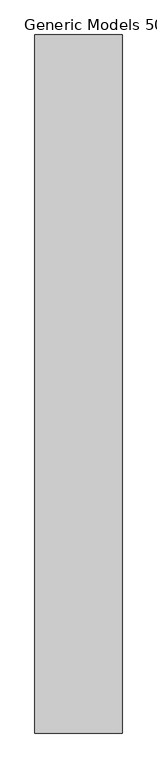
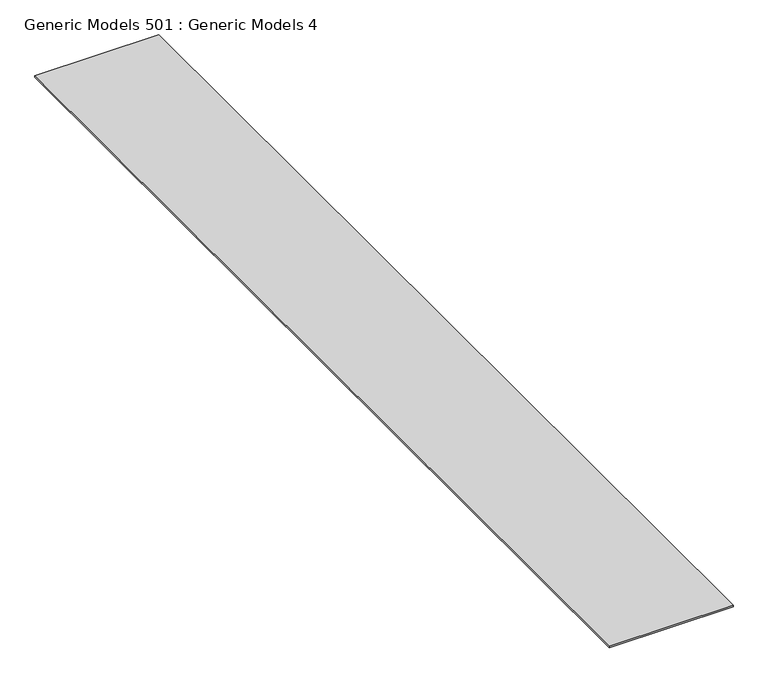
"""IFC4 building model written with IfcOpenShell, lengths in millimetres: proxy geometry, Generic Models 501 : Generic Models 4."""

import ifcopenshell
import ifcopenshell.guid

model = None  # the IFC model being written
_history = None  # IfcOwnerHistory: only IFC2X3 demands one
_inside = {}  # id of a spatial element -> (the spatial element, [elements in it])
_under = {}  # id of a project, library or spatial element -> (it, [spatial elements below it])
_declared = {}  # id of a project -> (the project, [libraries it declares])
_typed = {}  # id of a type object -> (the type object, [elements of that type])
_made_of = {}  # id of a material, layer set ... -> (it, [elements and type objects made of it])


def new_model(schema):
    """Start an empty IFC model of exactly this schema.

    Asked for "IFC4X3", IfcOpenShell would pick the latest addendum, in which some entities
    have other attributes; the version numbers below select the first issue.
    IFC2X3 requires an IfcOwnerHistory on every rooted entity: one is made here for all.
    """
    global model, _history
    if schema == "IFC4X3":
        model = ifcopenshell.file(schema_version=(4, 3, 0, 0))
    else:
        model = ifcopenshell.file(schema=schema)
    _inside.clear()
    _under.clear()
    _declared.clear()
    _typed.clear()
    _made_of.clear()
    _history = None
    if model.schema == "IFC2X3":
        org = make("IfcOrganization", Name="unknown")
        user = make(
            "IfcPersonAndOrganization",
            ThePerson=make("IfcPerson", FamilyName="unknown"),
            TheOrganization=org,
        )
        app = make(
            "IfcApplication",
            ApplicationDeveloper=org,
            Version="unknown",
            ApplicationFullName="unknown",
            ApplicationIdentifier="unknown",
        )
        _history = make(
            "IfcOwnerHistory",
            OwningUser=user,
            OwningApplication=app,
            ChangeAction="ADDED",
            CreationDate=0,
        )
    return model


def make(cls, **values):
    """One entity of the class cls with the attributes given. An attribute that is None is left unset."""
    return model.create_entity(
        cls, **{name: value for name, value in values.items() if value is not None}
    )


def rooted(cls, **values):
    """An entity with a GlobalId (a new one), such as an element, a storey or a relation."""
    return make(cls, GlobalId=ifcopenshell.guid.new(), OwnerHistory=_history, **values)


def si_unit(unit_type, name, prefix=None):
    """IfcSIUnit, for example si_unit("LENGTHUNIT", "METRE", prefix="MILLI")."""
    return make("IfcSIUnit", UnitType=unit_type, Prefix=prefix, Name=name)


def assignment(units):
    """IfcUnitAssignment: the units of a project."""
    return None if units is None else make("IfcUnitAssignment", Units=units)


def point(xyz):
    """IfcCartesianPoint."""
    return None if xyz is None else make("IfcCartesianPoint", Coordinates=xyz)


def direction(xyz):
    """IfcDirection."""
    return None if xyz is None else make("IfcDirection", DirectionRatios=xyz)


def frame(location, z_axis=None, x_axis=None):
    """IfcAxis2Placement3D, a coordinate frame: its origin and axes. An axis left out is left unset."""
    return make(
        "IfcAxis2Placement3D",
        Location=point(location),
        Axis=direction(z_axis),
        RefDirection=direction(x_axis),
    )


def origin():
    """The frame at (0, 0, 0) with its axes left unset."""
    return frame((0.0, 0.0, 0.0))


def place(relative_to, where):
    """IfcLocalPlacement: puts the frame where relative to a parent placement (None: the world)."""
    return make(
        "IfcLocalPlacement", PlacementRelTo=relative_to, RelativePlacement=where
    )


def context(
    kind, dimensions, precision=None, world=None, true_north=None, identifier=None
):
    """IfcGeometricRepresentationContext, for example the 3D "Model" context."""
    return make(
        "IfcGeometricRepresentationContext",
        ContextIdentifier=identifier,
        ContextType=kind,
        CoordinateSpaceDimension=dimensions,
        Precision=precision,
        WorldCoordinateSystem=world,
        TrueNorth=true_north,
    )


def project(units=None, contexts=None):
    """IfcProject with its units and contexts."""
    return rooted(
        "IfcProject",
        Name="project",
        RepresentationContexts=contexts,
        UnitsInContext=assignment(units),
    )


def spatial(cls, under=None, at=None, **own):
    """A site, building, storey or space (cls), placed at a placement, below another one or the project."""
    s = rooted(cls, ObjectPlacement=at, **own)
    if under is not None:
        _under.setdefault(under.id(), (under, []))[1].append(s)
    return s


def polyline(points):
    """IfcPolyline through the points."""
    return make("IfcPolyline", Points=[point(p) for p in points])


def outline(outer, holes=None, kind="AREA"):
    """IfcArbitraryClosedProfileDef: a profile drawn as a closed curve; with holes, ...WithVoids."""
    if holes is None:
        return make("IfcArbitraryClosedProfileDef", ProfileType=kind, OuterCurve=outer)
    return make(
        "IfcArbitraryProfileDefWithVoids",
        ProfileType=kind,
        OuterCurve=outer,
        InnerCurves=holes,
    )


def extrude(swept, where, along, depth):
    """IfcExtrudedAreaSolid: the profile swept, set in the frame where, extruded along a direction by depth."""
    return make(
        "IfcExtrudedAreaSolid",
        SweptArea=swept,
        Position=where,
        ExtrudedDirection=direction(along),
        Depth=depth,
    )


def shape(context_of_items, identifier, shape_type, items):
    """IfcShapeRepresentation: the items that make up one representation, for example the "Body"."""
    return make(
        "IfcShapeRepresentation",
        ContextOfItems=context_of_items,
        RepresentationIdentifier=identifier,
        RepresentationType=shape_type,
        Items=items,
    )


def source(mapping_origin, context_of_items, identifier, shape_type, items):
    """IfcRepresentationMap: a shape defined once, which mapped items show again and again."""
    return make(
        "IfcRepresentationMap",
        MappingOrigin=mapping_origin,
        MappedRepresentation=shape(context_of_items, identifier, shape_type, items),
    )


def transform(
    local_origin,
    x_axis=None,
    y_axis=None,
    z_axis=None,
    scale=None,
    scale2=None,
    scale3=None,
    uniform=True,
):
    """IfcCartesianTransformationOperator3D, or its non-uniform kind. x_axis, y_axis, z_axis: its Axis1, 2, 3."""
    if uniform:
        return make(
            "IfcCartesianTransformationOperator3D",
            Axis1=direction(x_axis),
            Axis2=direction(y_axis),
            LocalOrigin=point(local_origin),
            Scale=scale,
            Axis3=direction(z_axis),
        )
    return make(
        "IfcCartesianTransformationOperator3DnonUniform",
        Axis1=direction(x_axis),
        Axis2=direction(y_axis),
        LocalOrigin=point(local_origin),
        Scale=scale,
        Axis3=direction(z_axis),
        Scale2=scale2,
        Scale3=scale3,
    )


def mapped(mapping_source, mapping_target):
    """IfcMappedItem: shows the shape of a source again, moved by a transform."""
    return make(
        "IfcMappedItem", MappingSource=mapping_source, MappingTarget=mapping_target
    )


def made_of(thing, what):
    """Note that an element or type object is made of a material, layer set ...; save() writes the relation."""
    if what is not None:
        _made_of.setdefault(what.id(), (what, []))[1].append(thing)
    return thing


def element(
    cls,
    number,
    at=None,
    inside=None,
    cuts=None,
    type_object=None,
    material=None,
    context=None,
    identifier="Body",
    shape_type=None,
    held_by="IfcProductDefinitionShape",
    body=None,
    shapes=None,
    **own,
):
    """One element of the class cls, such as IfcWall. Its Tag is "e" and its number.

    at: its placement. inside: the storey or other place that contains it. cuts: it is an
    opening in that element (IfcRelVoidsElement). A single representation is given by context,
    identifier, shape_type and body (its items); several are given by shapes. held_by: the class
    of the entity that holds the representations. save() writes the other relations.
    """
    e = rooted(cls, Tag="e%d" % number, ObjectPlacement=at, **own)
    if body is not None:
        shapes = [shape(context, identifier, shape_type, body)]
    if shapes is not None:
        e.Representation = make(held_by, Representations=shapes)
    if inside is not None:
        _inside.setdefault(inside.id(), (inside, []))[1].append(e)
    if cuts is not None:
        rooted(
            "IfcRelVoidsElement", RelatingBuildingElement=cuts, RelatedOpeningElement=e
        )
    if type_object is not None:
        _typed.setdefault(type_object.id(), (type_object, []))[1].append(e)
    return made_of(e, material)


def aggregate(whole, parts):
    """IfcRelAggregates: a whole, such as a stair, and the parts it consists of."""
    return rooted("IfcRelAggregates", RelatingObject=whole, RelatedObjects=parts)


def save(model, path):
    """Write the relations noted so far, then the file.

    IfcRelAggregates (storeys below a building ...), IfcRelContainedInSpatialStructure (elements
    in a storey), IfcRelDefinesByType, IfcRelAssociatesMaterial and IfcRelDeclares: one each for
    every whole, place, type object, material and project.
    """
    for whole, parts in _under.values():
        aggregate(whole, parts)
    for where, things in _inside.values():
        rooted(
            "IfcRelContainedInSpatialStructure",
            RelatedElements=things,
            RelatingStructure=where,
        )
    for kind, things in _typed.values():
        rooted("IfcRelDefinesByType", RelatedObjects=things, RelatingType=kind)
    for what, things in _made_of.values():
        rooted("IfcRelAssociatesMaterial", RelatedObjects=things, RelatingMaterial=what)
    for by, libraries in _declared.values():
        rooted("IfcRelDeclares", RelatingContext=by, RelatedDefinitions=libraries)
    model.write(path)


def generic_models_501_generic_models_4_2ab117f4(model_context):
    return source(origin(), model_context, "Body", "SweptSolid", [
        extrude(outline(polyline([(-6629.5736296, -464.1230338), (-8156.7486296, -464.1230338), (-8156.7486296, 11778.6769662), (-6629.5736295, 11778.6769662), (-6629.5736296, -464.1230338)])), frame((0.0, 0.0, 126345.696), z_axis=(0.0, 0.0, 1.0), x_axis=(1.0, 0.0, 0.0)), (0.0, 0.0, 1.0), 19.05),
    ])


if __name__ == "__main__":
    model = new_model("IFC4")
    model_context = context("Model", 3, world=origin())
    ifc_project = project(units=[si_unit("LENGTHUNIT", "METRE", prefix="MILLI")], contexts=[model_context])
    site = spatial("IfcSite", under=ifc_project)
    building = spatial("IfcBuilding", under=site)
    placement = place(None, origin())
    generic_models_501_generic_models_4_shape = generic_models_501_generic_models_4_2ab117f4(model_context)
    element("IfcBuildingElementProxy", 1, Name="Generic Models 501 : Generic Models 4", ObjectType="Generic Models 501 : Generic Models 4", at=placement, inside=building, context=model_context, shape_type="MappedRepresentation", body=[
        mapped(generic_models_501_generic_models_4_shape, transform((0.0, 0.0, 0.0), x_axis=(1.0, 0.0, 0.0), y_axis=(0.0, 1.0, 0.0), z_axis=(0.0, 0.0, 1.0))),
    ])
    save(model, "model.ifc")

# Revit data of these elements
# Element 1 (IfcBuildingElementProxy, "Generic Models 501 : Generic Models 4")
#   Materials on its faces: "_T&G FIRE RETARDANT WOOD SOFFIT O/ BUILDING PAPER"
# Materials
#   "_T&G FIRE RETARDANT WOOD SOFFIT O/ BUILDING PAPER": class "Generic", colour RGB 177 130 114, transparency 0, Cost = 0
